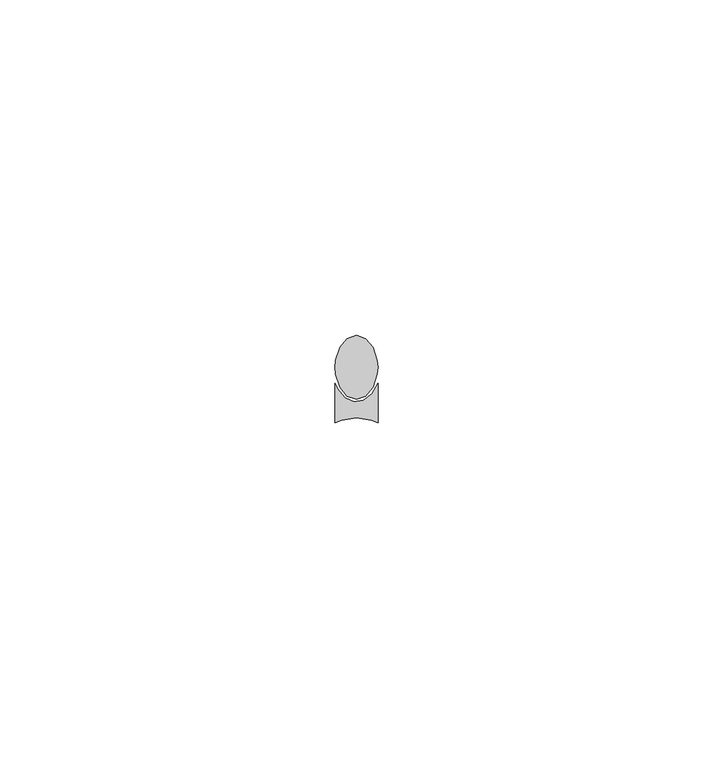
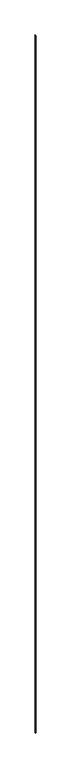
"""IFC4 building model written with IfcOpenShell, lengths in millimetres: proxy geometry, Generic Models 11:Generic Models 1:306267:Generic Models 1:306267 : Generic Models 11:Generic Models 1:306267:300405:Generic Models 1:306267:Generic Models 1:306267 : Generic Models 11:Generic Models 1:306267:300405 : Generic Models 11:Generic Models 1:306267:Generic Models 1:306267 : Generic Models 11:Generic Models 1:306267:300405:21 : Generic Models 11:Generic Models 1:306267:Generic Models 1:306267 : Generic Models 11:Generic Models 1:306267:300405:Generic Models 1:306267:Generic Models 1:306267 : Generic Models 11:Generic Models 1:306267:300405 : Generic Models 11:Generic Models 1:306267:Generic Models 1:306267 : Generic Models 11:Generic Models 1:306267:300405:300182."""

from ifc_helpers import new_model, si_unit, origin, origin_with_axes, place, context, project, spatial, polyline, outline, extrude, source, transform, mapped, element, save


def generic_models_dd902c01(model_context):
    return source(origin(), model_context, "Body", "SweptSolid", [
        extrude(outline(polyline([(593733.5341431, -579092.0005286), (593732.429409, -579090.6790346), (593731.8163278, -579088.7694203), (593731.7367239, -579087.7096644), (593731.8163278, -579086.6499084), (593732.429409, -579084.7402942), (593733.5341431, -579083.4188002), (593734.9117239, -579082.9471644), (593736.2893048, -579083.4188002), (593737.3940389, -579084.7402942), (593738.0071201, -579086.6499084), (593738.0867239, -579087.7096644), (593738.0071201, -579088.7694203), (593737.3940389, -579090.6790346), (593736.2893048, -579092.0005286), (593734.9117239, -579092.4721644), (593733.5341431, -579092.0005286)])), origin_with_axes(), (0.0, 0.0, 1.0), 8555.7679991),
        extrude(outline(polyline([(593737.1209607, -579095.5639755), (593734.9117239, -579095.2502894), (593732.7024872, -579095.5639755), (593731.7367239, -579095.9413841), (593731.7367239, -579090.073292), (593732.1230415, -579090.9335729), (593733.206527, -579092.2431481), (593734.5567747, -579092.8435016), (593735.962551, -579092.6407137), (593737.2039351, -579091.6665087), (593738.0867239, -579090.073292), (593738.0867239, -579095.9413841), (593737.1209607, -579095.5639755)])), origin_with_axes(), (0.0, 0.0, 1.0), 8555.7679991),
    ])


if __name__ == "__main__":
    model = new_model("IFC4")
    model_context = context("Model", 3, world=origin())
    ifc_project = project(units=[si_unit("LENGTHUNIT", "METRE", prefix="MILLI")], contexts=[model_context])
    site = spatial("IfcSite", under=ifc_project)
    building = spatial("IfcBuilding", under=site)
    placement = place(None, origin())
    generic_models_shape = generic_models_dd902c01(model_context)
    element("IfcBuildingElementProxy", 1, Name="Generic Models 11:Generic Models 1:306267:Generic Models 1:306267 : Generic Models 11:Generic Models 1:306267:300405:Generic Models 1:306267:Generic Models 1:306267 : Generic Models 11:Generic Models 1:306267:300405 : Generic Models 11:Generic Models 1:306267:Generic Models 1:306267 : Generic Models 11:Generic Models 1:306267:300405:21 : Generic Models 11:Generic Models 1:306267:Generic Models 1:306267 : Generic Models 11:Generic Models 1:306267:300405:Generic Models 1:306267:Generic Models 1:306267 : Generic Models 11:Generic Models 1:306267:300405 : Generic Models 11:Generic Models 1:306267:Generic Models 1:306267 : Generic Models 11:Generic Models 1:306267:300405:300182", ObjectType="Generic Models 11:Generic Models 1:306267:Generic Models 1:306267 : Generic Models 11:Generic Models 1:306267:300405:Generic Models 1:306267:Generic Models 1:306267 : Generic Models 11:Generic Models 1:306267:300405 : Generic Models 11:Generic Models 1:306267:Generic Models 1:306267 : Generic Models 11:Generic Models 1:306267:300405:21 : Generic Models 11:Generic Models 1:306267:Generic Models 1:306267 : Generic Models 11:Generic Models 1:306267:300405:Generic Models 1:306267:Generic Models 1:306267 : Generic Models 11:Generic Models 1:306267:300405 : Generic Models 11:Generic Models 1:306267:Generic Models 1:306267 : Generic Models 11:Generic Models 1:306267:300405:300182", at=placement, inside=building, context=model_context, shape_type="MappedRepresentation", body=[
        mapped(generic_models_shape, transform((0.0, 0.0, 0.0), x_axis=(1.0, 0.0, 0.0), y_axis=(0.0, 1.0, 0.0), z_axis=(0.0, 0.0, 1.0))),
    ])
    save(model, "model.ifc")

# Revit data of these elements
# Type "Generic Models 11:Generic Models 1:306267:Generic Models 1:306267 : Generic Models 11:Generic Models 1:306267:300405:Generic Models 1:306267:Generic Models 1:306267 : Generic Models 11:Generic Models 1:306267:300405 : Generic Models 11:Generic Models 1:306267:Generic Models 1:306267 : Generic Models 11:Generic Models 1:306267:300405:21 : Generic Models 11:Generic Models 1:306267:Generic Models 1:306267 : Generic Models 11:Generic Models 1:306267:300405:Generic Models 1:306267:Generic Models 1:306267 : Generic Models 11:Generic Models 1:306267:300405 : Generic Models 11:Generic Models 1:306267:Generic Models 1:306267 : Generic Models 11:Generic Models 1:306267:300405:300182"
#   NameOverride = "Generic Models 11:Generic Models 1:306267:Generic Models 1:306267 : Generic Models 11:Generic Models 1:306267:300405:Generic Models 1:306267:Generic Models 1:306267 : Generic Models 11:Generic Models 1:306267:300405 : Generic Models 11:Generic Models 1:306267:Generic Models 1:306267 : Generic Models 11:Generic Models 1:306267:300405:300182"
#   ObjectTypeOverride = "Generic Models 1:306267:Generic Models 1:306267 : Generic Models 11:Generic Models 1:306267:300405 : Generic Models 11:Generic Models 1:306267:Generic Models 1:306267 : Generic Models 11:Generic Models 1:306267:300405"
#   Reference = "Generic Models 1"
#   Tag = "300182"
# Element 1 (IfcBuildingElementProxy, "Generic Models 11:Generic Models 1:306267:Generic Models 1:306267 : Generic Models 11:Generic Models 1:306267:300405:Generic Models 1:306267:Generic Models 1:306267 : Generic Models 11:Generic Models 1:306267:300405 : Generic Models 11:Generic Models 1:306267:Generic Models 1:306267 : Generic Models 11:Generic Models 1:306267:300405:21 : Generic Models 11:Generic Models 1:306267:Generic Models 1:306267 : Generic Models 11:Generic Models 1:306267:300405:Generic Models 1:306267:Generic Models 1:306267 : Generic Models 11:Generic Models 1:306267:300405 : Generic Models 11:Generic Models 1:306267:Generic Models 1:306267 : Generic Models 11:Generic Models 1:306267:300405:300182")
#   Materials on its faces: "SEALANT & BACKER ROD"
# Materials
#   "SEALANT & BACKER ROD": class "Unassigned", colour RGB 120 120 120, transparency 0, Cost = 0
